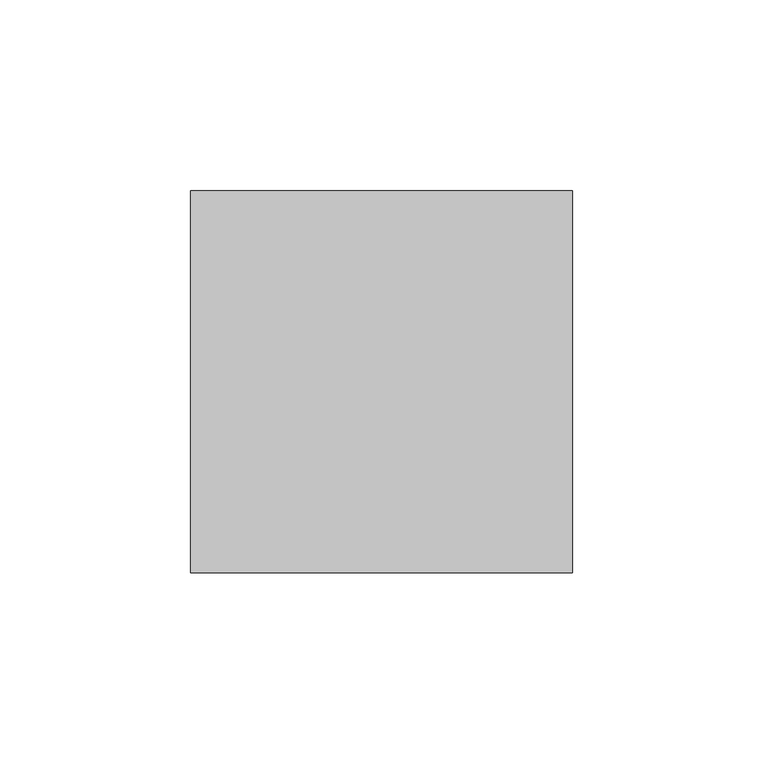
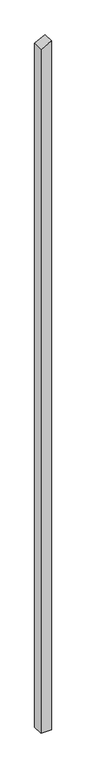
"""IFC4 building model written with IfcOpenShell, lengths in millimetres: column geometry, Holzstütze 159856 : Holzstütze 159856."""

from ifc_helpers import new_model, si_unit, frame, origin, place, context, project, spatial, polyline, outline, extrude, source, transform, mapped, element, save


def column_93f356e6(model_context):
    return source(origin(), model_context, "Body", "SweptSolid", [
        extrude(outline(polyline([(-500.0, 157297.7593015), (-500.0, 157397.7593015), (6396.6643707, 157397.7593015), (6345.7118258, 157297.7593015), (-500.0, 157297.7593015)])), frame((0.0, 39349.3988814, 0.0), z_axis=(0.0, 1.0, 0.0), x_axis=(0.0, 0.0, 1.0)), (0.0, 0.0, 1.0), 100.0),
    ])


if __name__ == "__main__":
    model = new_model("IFC4")
    model_context = context("Model", 3, world=origin())
    ifc_project = project(units=[si_unit("LENGTHUNIT", "METRE", prefix="MILLI")], contexts=[model_context])
    site = spatial("IfcSite", under=ifc_project)
    building = spatial("IfcBuilding", under=site)
    placement = place(None, origin())
    column_shape = column_93f356e6(model_context)
    element("IfcColumn", 1, ObjectType="Holzstütze 159856 : Holzstütze 159856", at=placement, inside=building, context=model_context, shape_type="MappedRepresentation", body=[
        mapped(column_shape, transform((0.0, 0.0, 0.0), x_axis=(1.0, 0.0, 0.0), y_axis=(0.0, 1.0, 0.0), z_axis=(0.0, 0.0, 1.0))),
    ])
    save(model, "model.ifc")

# Revit data of these elements
# Type "Holzstütze 159856 : Holzstütze 159856"
#   Abrechnungsart = "m"
#   Allright_Bauteil_ID = "0152St 0000143512"
#   Bezeichnung = "Holzstütze"
#   Codetext = "ST-HOLZ\\"
#   Gewerk = "Zimmer- und Holzbauarbeiten"
#   Material = "Holz"
#   Objektname = "Stütze"
#   NameOverride = "Holzstütze"
#   Reference = "Holzstütze"
#   Status = "NEW"
#   ThermalTransmittance = 0.0000 BTU/(h·ft²·°F)
#   Roll = 0.00°
#   Slope = 0.00°
#   2D Interaktion = yes
#   IsExternal = yes
#   LoadBearing = yes
# Element 1 (IfcColumn, "Holzstütze 159856 : Holzstütze 159856")
#   Materials on its faces: "holzschalung"
# Materials
#   "holzschalung": class "Unassigned", colour RGB 128 128 128, transparency 0
